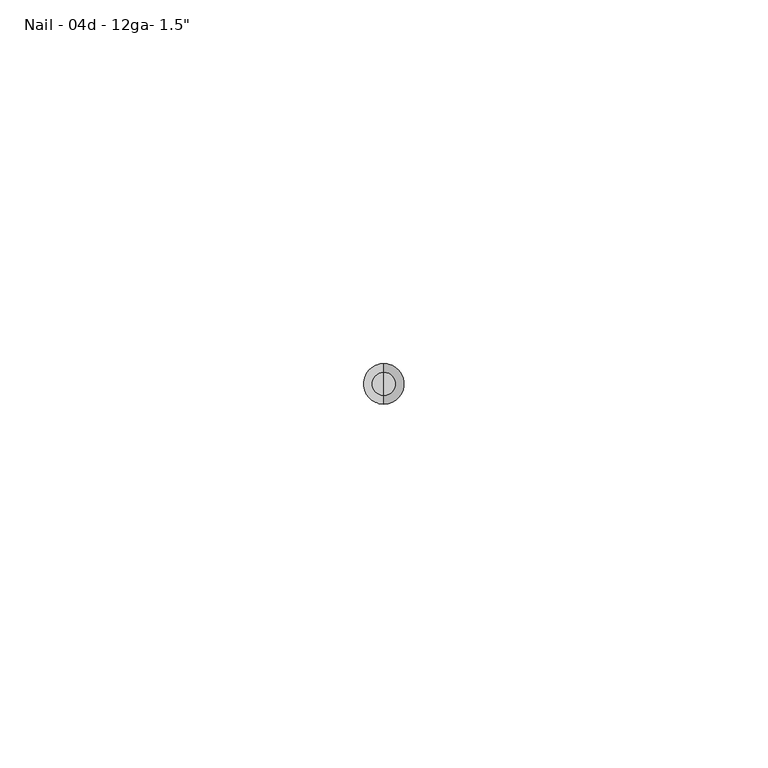
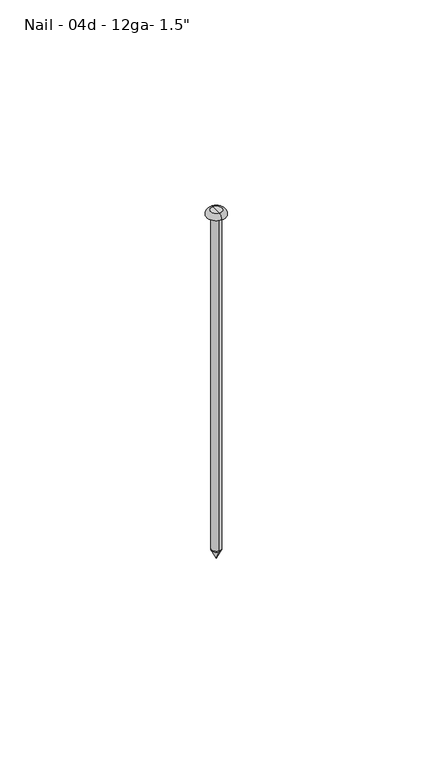
"""IFC4 building model written with IfcOpenShell, lengths in millimetres: fastener geometry."""

from ifc_helpers import new_model, si_unit, point, frame, origin, origin_2d, place, context, project, spatial, polyline, circle_curve, ellipse_curve, trimmed, segment, composite_curve, outline, extrude, source, transform, mapped, element, save
from ifc_brep_helpers import plane_surface, revolved_surface, advanced_brep


def fastener_6e0a6073(model_context):
    return source(origin(), model_context, "Body", "SolidModel", [
        advanced_brep(
        [(0.0, -1.3843, -101.6), (0.0, 1.3843, -101.6), (0.0, 0.0, -101.6), (0.0, 0.0, -104.3686)],
        [
            (0, 1, circle_curve(frame((0.0, 0.0, -101.6), z_axis=(0.0, 0.0, 1.0), x_axis=(0.0, 1.0, 0.0)), 1.3843)),
            (1, 2),
            (2, 0),
            (1, 0, circle_curve(frame((0.0, 0.0, -101.6), z_axis=(0.0, 0.0, 1.0), x_axis=(0.0, 1.0, 0.0)), 1.3843)),
            (3, 1),
            (0, 3),
        ],
        [
            plane_surface(frame((0.0, 0.0, -101.6), z_axis=(0.0, 0.0, 1.0), x_axis=(0.0, 1.0, 0.0))),
            revolved_surface(polyline([(0.0, 1.3843, -101.6), (0.0, 0.0, -104.3686)]), (0.0, 0.0, -103.0840259), (0.0, 0.0, -1.0)),
        ],
        [
            (0, [[1, 2, 3]]),
            (0, [[4, -3, -2]]),
            (1, [[5, -1, 6]]),
            (1, [[-6, -4, -5]]),
        ],
    ),
        advanced_brep(
        [(0.0, 2.7686, 0.0), (0.0, -2.7686, 0.0), (0.0, 0.0, 0.0), (0.0, 0.0, 1.3843), (0.0, -1.5875, 1.3843), (0.0, 1.5875, 1.3843)],
        [
            (0, 1, circle_curve(frame((0.0, 0.0, 0.0), z_axis=(0.0, 0.0, -1.0), x_axis=(0.0, -1.0, 0.0)), 2.7686)),
            (1, 2),
            (2, 0),
            (1, 0, circle_curve(frame((0.0, 0.0, 0.0), z_axis=(0.0, 0.0, -1.0), x_axis=(0.0, -1.0, 0.0)), 2.7686)),
            (3, 4),
            (4, 5, circle_curve(frame((0.0, 0.0, 1.3843), z_axis=(0.0, 0.0, 1.0), x_axis=(0.0, -1.0, 0.0)), 1.5875)),
            (5, 3),
            (5, 4, circle_curve(frame((0.0, 0.0, 1.3843), z_axis=(0.0, 0.0, 1.0), x_axis=(0.0, -1.0, 0.0)), 1.5875)),
            (4, 1, circle_curve(frame((0.0, -1.5875, 0.1882862), z_axis=(1.0, 0.0, 0.0), x_axis=(0.0, -1.0, 0.0)), 1.1960138)),
            (0, 5, circle_curve(frame((0.0, 1.5875, 0.1882862), z_axis=(1.0, 0.0, 0.0), x_axis=(0.0, 1.0, 0.0)), 1.1960138)),
        ],
        [
            plane_surface(frame((0.0, 0.0, 0.0), z_axis=(0.0, 0.0, -1.0), x_axis=(0.0, -1.0, 0.0))),
            plane_surface(frame((0.0, 0.0, 1.3843), z_axis=(0.0, 0.0, 1.0), x_axis=(0.0, -1.0, 0.0))),
            revolved_surface(trimmed(ellipse_curve(frame((0.0, -1.5875, 0.1882862), z_axis=(-1.0, 0.0, 0.0), x_axis=(0.0, -1.0, 0.0)), 1.1960138, 1.1960138), [point((0.0, -2.7686, 0.0))], [point((0.0, -1.5875, 1.3843))], True, "CARTESIAN"), (0.0, 0.0, 1.4840259), (0.0, 0.0, 1.0)),
        ],
        [
            (0, [[1, 2, 3]]),
            (0, [[4, -3, -2]]),
            (1, [[5, 6, 7]]),
            (1, [[-7, 8, -5]]),
            (2, [[-6, 9, -1, 10]]),
            (2, [[-8, -10, -4, -9]]),
        ],
    ),
        extrude(outline(composite_curve([segment(trimmed(circle_curve(origin_2d(), 1.3843), [point((0.0, -1.3843))], [point((0.0, 1.3843))], False, "CARTESIAN"), True, "CONTINUOUS"), segment(trimmed(circle_curve(origin_2d(), 1.3843), [point((0.0, 1.3843))], [point((0.0, -1.3843))], False, "CARTESIAN"), True, "CONTINUOUS")], self_intersect=False)), frame((0.0, 0.0, -101.6), z_axis=(0.0, 0.0, 1.0), x_axis=(1.0, 0.0, 0.0)), (0.0, 0.0, 1.0), 101.6),
    ])


if __name__ == "__main__":
    model = new_model("IFC4")
    model_context = context("Model", 3, world=origin())
    ifc_project = project(units=[si_unit("LENGTHUNIT", "METRE", prefix="MILLI")], contexts=[model_context])
    site = spatial("IfcSite", under=ifc_project)
    building = spatial("IfcBuilding", under=site)
    placement = place(None, origin())
    fastener_shape = fastener_6e0a6073(model_context)
    element("IfcFastener", 1, ObjectType="060523 - W_P_C - Fastenings - Generic : Nail - 04d - 12ga- 1.5\"", at=placement, inside=building, context=model_context, shape_type="MappedRepresentation", body=[
        mapped(fastener_shape, transform((0.0, 0.0, 0.0), x_axis=(1.0, 0.0, 0.0), y_axis=(0.0, 1.0, 0.0), z_axis=(0.0, 0.0, 1.0))),
    ])
    save(model, "model.ifc")

# Revit data of these elements
# Type "060523 - W_P_C - Fastenings - Generic : Nail - 04d - 12ga- 1.5\""
#   Washer_Thickness = 0' - 0.00333"
#   Washer Radius = 0' - 0.0645"
#   Washer Offset - Head = 0' - 0"
#   Washer Offset = 0' - 0"
#   Thickness_of_Substrate [instance default] = 0' - 1"
#   Side = 0' - 0 37/64"
#   Radius = 0' - 0.0545"
#   Length [instance default] = 0' - 1 1/2"
#   Head Size = 0' - 1"
#   Head Radius = 0' - 0 1/2"
#   Head Height = 0' - 0.01"
#   Double Diameter = 0' - 0.218"
#   Diameter = 0' - 0.109"
#   Default Elevation = 4' - 0"
#   Washer_Nut_Visibility = no
#   Washer_Head_Visibility = no
#   Round_Head_Visibility = yes
#   Point Visibility = yes
#   Nut_Visibility = no
#   Hex_Head_Visiblilty = no
#   Washer Material = none
#   Bolt Material (Size) = AT SILL - FASTENER AT 24" O.C.
# Element 1 (IfcFastener, "060523 - W_P_C - Fastenings - Generic : Nail - 04d - 12ga- 1.5\"")
#   Length = 0' - 4"
#   Materials on its faces: "AT SILL - FASTENER AT 24\" O.C."
# Materials
#   "AT SILL - FASTENER AT 24\" O.C.": class "Generic", colour RGB 120 120 120, transparency 0, Cost = 0
